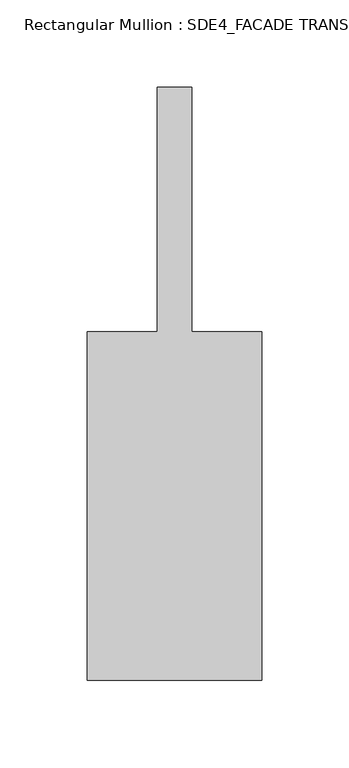
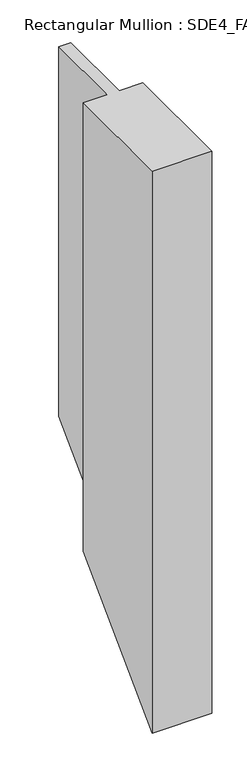
"""IFC4 building model written with IfcOpenShell, lengths in millimetres: member geometry, Rectangular Mullion : SDE4_FACADE TRANSOM TYPE 1."""

from ifc_helpers import new_model, si_unit, origin, place, context, project, spatial, faceted_brep, source, transform, mapped, element, save


def rectangular_mullion_sde4_facade_transom_type_1_f0cdf0ef(model_context):
    return source(origin(), model_context, "Body", "Brep", [
        faceted_brep([(50.0, -132.5, 0.0), (50.0, 67.5, 0.0), (10.0, 67.5, 0.0), (10.0, 207.5, 0.0), (-10.0, 207.5, 0.0), (-10.0, 67.5, 0.0), (-50.0, 67.5, 0.0), (-50.0, -132.5, 0.0), (50.0, -132.5, -994.0375289), (50.0, 67.5, -794.0375289), (10.0, 67.5, -794.0375289), (10.0, 207.5, -654.0375289), (-10.0, 207.5, -654.0375289), (-10.0, 67.5, -794.0375289), (-50.0, 67.5, -794.0375289), (-50.0, -132.5, -994.0375289)], [[[0, 1, 2, 3, 4, 5, 6, 7]], [[1, 0, 8, 9]], [[2, 1, 9, 10]], [[3, 2, 10, 11]], [[4, 3, 11, 12]], [[5, 4, 12, 13]], [[6, 5, 13, 14]], [[7, 6, 14, 15]], [[0, 7, 15, 8]], [[8, 15, 14, 13, 12, 11, 10, 9]]]),
    ])


if __name__ == "__main__":
    model = new_model("IFC4")
    model_context = context("Model", 3, world=origin())
    ifc_project = project(units=[si_unit("LENGTHUNIT", "METRE", prefix="MILLI")], contexts=[model_context])
    site = spatial("IfcSite", under=ifc_project)
    building = spatial("IfcBuilding", under=site)
    placement = place(None, origin())
    rectangular_mullion_sde4_facade_transom_type_1_shape = rectangular_mullion_sde4_facade_transom_type_1_f0cdf0ef(model_context)
    element("IfcMember", 1, ObjectType="Rectangular Mullion : SDE4_FACADE TRANSOM TYPE 1", at=placement, inside=building, context=model_context, shape_type="MappedRepresentation", body=[
        mapped(rectangular_mullion_sde4_facade_transom_type_1_shape, transform((0.0, 0.0, 0.0), x_axis=(1.0, 0.0, 0.0), y_axis=(0.0, 1.0, 0.0), z_axis=(0.0, 0.0, 1.0))),
    ])
    save(model, "model.ifc")

# Revit data of these elements
# Type "Rectangular Mullion : SDE4_FACADE TRANSOM TYPE 1"
#   built-in parameter 1007322 = 1.11549 (stored number, unit not read)
#   built-in parameter 1007321 = 0.164042 (stored number, unit not read)
#   built-in parameter 1007320 = 0.164042 (stored number, unit not read)
